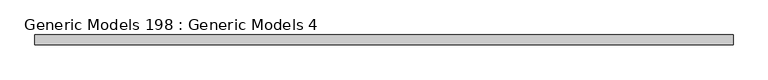
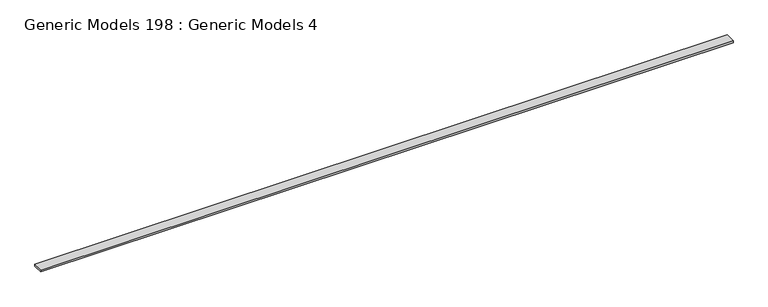
"""IFC4 building model written with IfcOpenShell, lengths in millimetres: proxy geometry, Generic Models 198 : Generic Models 4."""

from ifc_helpers import new_model, si_unit, frame, origin, place, context, project, spatial, polyline, outline, extrude, source, transform, mapped, element, save


def generic_models_198_generic_models_4_6b4c619b(model_context):
    return source(origin(), model_context, "Body", "SweptSolid", [
        extrude(outline(polyline([(-25153.2674751, 127104.4735933), (-25331.0674751, 127104.4735933), (-25331.0674751, 127136.7527599), (-25153.2674751, 127144.1610933), (-25153.2674751, 127104.4735933)])), frame((-20795.7733045, 0.0, 0.0), z_axis=(1.0, 0.0, 0.0), x_axis=(0.0, 1.0, 0.0)), (0.0, 0.0, 1.0), 12453.668502),
    ])


if __name__ == "__main__":
    model = new_model("IFC4")
    model_context = context("Model", 3, world=origin())
    ifc_project = project(units=[si_unit("LENGTHUNIT", "METRE", prefix="MILLI")], contexts=[model_context])
    site = spatial("IfcSite", under=ifc_project)
    building = spatial("IfcBuilding", under=site)
    placement = place(None, origin())
    generic_models_198_generic_models_4_shape = generic_models_198_generic_models_4_6b4c619b(model_context)
    element("IfcBuildingElementProxy", 1, Name="Generic Models 198 : Generic Models 4", ObjectType="Generic Models 198 : Generic Models 4", at=placement, inside=building, context=model_context, shape_type="MappedRepresentation", body=[
        mapped(generic_models_198_generic_models_4_shape, transform((0.0, 0.0, 0.0), x_axis=(1.0, 0.0, 0.0), y_axis=(0.0, 1.0, 0.0), z_axis=(0.0, 0.0, 1.0))),
    ])
    save(model, "model.ifc")

# Revit data of these elements
# Element 1 (IfcBuildingElementProxy, "Generic Models 198 : Generic Models 4")
#   Materials on its faces: "_2X BLOCKING AS REQUIRED"
# Materials
#   "_2X BLOCKING AS REQUIRED": class "Generic", colour RGB 177 130 114, transparency 0, Cost = 0
